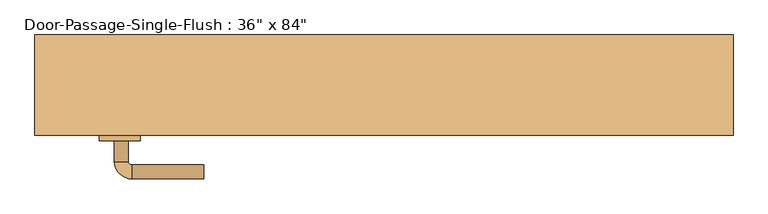
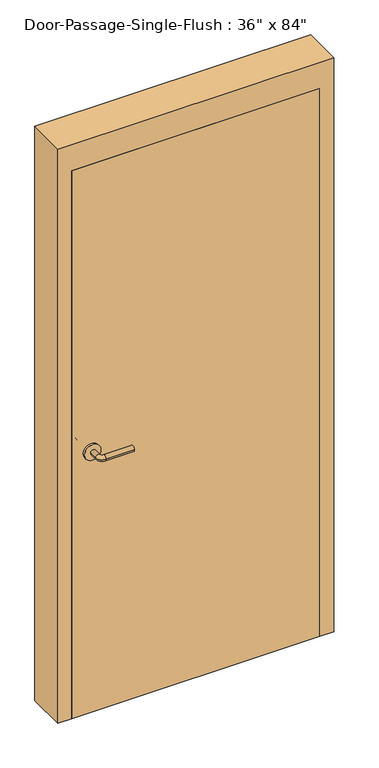
"""IFC4 building model written with IfcOpenShell, lengths in millimetres: door geometry."""

import ifcopenshell
import ifcopenshell.guid

model = None  # the IFC model being written
_history = None  # IfcOwnerHistory: only IFC2X3 demands one
_inside = {}  # id of a spatial element -> (the spatial element, [elements in it])
_under = {}  # id of a project, library or spatial element -> (it, [spatial elements below it])
_declared = {}  # id of a project -> (the project, [libraries it declares])
_typed = {}  # id of a type object -> (the type object, [elements of that type])
_made_of = {}  # id of a material, layer set ... -> (it, [elements and type objects made of it])


def new_model(schema):
    """Start an empty IFC model of exactly this schema.

    Asked for "IFC4X3", IfcOpenShell would pick the latest addendum, in which some entities
    have other attributes; the version numbers below select the first issue.
    IFC2X3 requires an IfcOwnerHistory on every rooted entity: one is made here for all.
    """
    global model, _history
    if schema == "IFC4X3":
        model = ifcopenshell.file(schema_version=(4, 3, 0, 0))
    else:
        model = ifcopenshell.file(schema=schema)
    _inside.clear()
    _under.clear()
    _declared.clear()
    _typed.clear()
    _made_of.clear()
    _history = None
    if model.schema == "IFC2X3":
        org = make("IfcOrganization", Name="unknown")
        user = make(
            "IfcPersonAndOrganization",
            ThePerson=make("IfcPerson", FamilyName="unknown"),
            TheOrganization=org,
        )
        app = make(
            "IfcApplication",
            ApplicationDeveloper=org,
            Version="unknown",
            ApplicationFullName="unknown",
            ApplicationIdentifier="unknown",
        )
        _history = make(
            "IfcOwnerHistory",
            OwningUser=user,
            OwningApplication=app,
            ChangeAction="ADDED",
            CreationDate=0,
        )
    return model


def make(cls, **values):
    """One entity of the class cls with the attributes given. An attribute that is None is left unset."""
    return model.create_entity(
        cls, **{name: value for name, value in values.items() if value is not None}
    )


def rooted(cls, **values):
    """An entity with a GlobalId (a new one), such as an element, a storey or a relation."""
    return make(cls, GlobalId=ifcopenshell.guid.new(), OwnerHistory=_history, **values)


def si_unit(unit_type, name, prefix=None):
    """IfcSIUnit, for example si_unit("LENGTHUNIT", "METRE", prefix="MILLI")."""
    return make("IfcSIUnit", UnitType=unit_type, Prefix=prefix, Name=name)


def assignment(units):
    """IfcUnitAssignment: the units of a project."""
    return None if units is None else make("IfcUnitAssignment", Units=units)


def point(xyz):
    """IfcCartesianPoint."""
    return None if xyz is None else make("IfcCartesianPoint", Coordinates=xyz)


def direction(xyz):
    """IfcDirection."""
    return None if xyz is None else make("IfcDirection", DirectionRatios=xyz)


def frame(location, z_axis=None, x_axis=None):
    """IfcAxis2Placement3D, a coordinate frame: its origin and axes. An axis left out is left unset."""
    return make(
        "IfcAxis2Placement3D",
        Location=point(location),
        Axis=direction(z_axis),
        RefDirection=direction(x_axis),
    )


def frame_2d(location, x_axis=None):
    """IfcAxis2Placement2D, a coordinate frame in the plane: its origin and x axis."""
    return make(
        "IfcAxis2Placement2D", Location=point(location), RefDirection=direction(x_axis)
    )


def origin():
    """The frame at (0, 0, 0) with its axes left unset."""
    return frame((0.0, 0.0, 0.0))


def origin_with_axes():
    """The frame at (0, 0, 0) with the z axis (0, 0, 1) and the x axis (1, 0, 0) written out."""
    return frame((0.0, 0.0, 0.0), z_axis=(0.0, 0.0, 1.0), x_axis=(1.0, 0.0, 0.0))


def place(relative_to, where):
    """IfcLocalPlacement: puts the frame where relative to a parent placement (None: the world)."""
    return make(
        "IfcLocalPlacement", PlacementRelTo=relative_to, RelativePlacement=where
    )


def context(
    kind, dimensions, precision=None, world=None, true_north=None, identifier=None
):
    """IfcGeometricRepresentationContext, for example the 3D "Model" context."""
    return make(
        "IfcGeometricRepresentationContext",
        ContextIdentifier=identifier,
        ContextType=kind,
        CoordinateSpaceDimension=dimensions,
        Precision=precision,
        WorldCoordinateSystem=world,
        TrueNorth=true_north,
    )


def project(units=None, contexts=None):
    """IfcProject with its units and contexts."""
    return rooted(
        "IfcProject",
        Name="project",
        RepresentationContexts=contexts,
        UnitsInContext=assignment(units),
    )


def spatial(cls, under=None, at=None, **own):
    """A site, building, storey or space (cls), placed at a placement, below another one or the project."""
    s = rooted(cls, ObjectPlacement=at, **own)
    if under is not None:
        _under.setdefault(under.id(), (under, []))[1].append(s)
    return s


def polyline(points):
    """IfcPolyline through the points."""
    return make("IfcPolyline", Points=[point(p) for p in points])


def circle_curve(where, radius):
    """IfcCircle in the frame where."""
    return make("IfcCircle", Position=where, Radius=radius)


def ellipse_curve(where, semi_axis1, semi_axis2):
    """IfcEllipse in the frame where."""
    return make(
        "IfcEllipse", Position=where, SemiAxis1=semi_axis1, SemiAxis2=semi_axis2
    )


def trimmed(basis, trim1, trim2, sense, master):
    """IfcTrimmedCurve: the piece of a basis curve between two trims."""
    return make(
        "IfcTrimmedCurve",
        BasisCurve=basis,
        Trim1=trim1,
        Trim2=trim2,
        SenseAgreement=sense,
        MasterRepresentation=master,
    )


def segment(curve, same_sense, transition):
    """IfcCompositeCurveSegment."""
    return make(
        "IfcCompositeCurveSegment",
        Transition=transition,
        SameSense=same_sense,
        ParentCurve=curve,
    )


def composite_curve(segments, self_intersect=None):
    """IfcCompositeCurve: segments joined end to end."""
    return make("IfcCompositeCurve", Segments=segments, SelfIntersect=self_intersect)


def outline(outer, holes=None, kind="AREA"):
    """IfcArbitraryClosedProfileDef: a profile drawn as a closed curve; with holes, ...WithVoids."""
    if holes is None:
        return make("IfcArbitraryClosedProfileDef", ProfileType=kind, OuterCurve=outer)
    return make(
        "IfcArbitraryProfileDefWithVoids",
        ProfileType=kind,
        OuterCurve=outer,
        InnerCurves=holes,
    )


def extrude(swept, where, along, depth):
    """IfcExtrudedAreaSolid: the profile swept, set in the frame where, extruded along a direction by depth."""
    return make(
        "IfcExtrudedAreaSolid",
        SweptArea=swept,
        Position=where,
        ExtrudedDirection=direction(along),
        Depth=depth,
    )


def faces_of(points, faces, orient=None, outer=None):
    """IfcFace entities. A face is a list of loops; a loop is a list of indices into points, from 0.

    orient and outer hold one flag for each loop. By default every Orientation is true, the
    first loop of a face is its IfcFaceOuterBound and the others are IfcFaceBound.
    """
    made = []
    for i, loops in enumerate(faces):
        bounds = []
        for j, loop in enumerate(loops):
            is_outer = j == 0 if outer is None else outer[i][j]
            bounds.append(
                make(
                    "IfcFaceOuterBound" if is_outer else "IfcFaceBound",
                    Bound=make("IfcPolyLoop", Polygon=[points[k] for k in loop]),
                    Orientation=True if orient is None else orient[i][j],
                )
            )
        made.append(make("IfcFace", Bounds=bounds))
    return made


def faceted_brep(points, faces, orient=None, outer=None, voids=None):
    """IfcFacetedBrep: a solid bounded by flat faces; with voids (closed shells), ...WithVoids."""
    shared = [point(p) for p in points]
    hull = make("IfcClosedShell", CfsFaces=faces_of(shared, faces, orient, outer))
    if voids is None:
        return make("IfcFacetedBrep", Outer=hull)
    return make(
        "IfcFacetedBrepWithVoids",
        Outer=hull,
        Voids=[
            make(cls, CfsFaces=faces_of(shared, fs, o, b)) for cls, fs, o, b in voids
        ],
    )


def shape(context_of_items, identifier, shape_type, items):
    """IfcShapeRepresentation: the items that make up one representation, for example the "Body"."""
    return make(
        "IfcShapeRepresentation",
        ContextOfItems=context_of_items,
        RepresentationIdentifier=identifier,
        RepresentationType=shape_type,
        Items=items,
    )


def source(mapping_origin, context_of_items, identifier, shape_type, items):
    """IfcRepresentationMap: a shape defined once, which mapped items show again and again."""
    return make(
        "IfcRepresentationMap",
        MappingOrigin=mapping_origin,
        MappedRepresentation=shape(context_of_items, identifier, shape_type, items),
    )


def transform(
    local_origin,
    x_axis=None,
    y_axis=None,
    z_axis=None,
    scale=None,
    scale2=None,
    scale3=None,
    uniform=True,
):
    """IfcCartesianTransformationOperator3D, or its non-uniform kind. x_axis, y_axis, z_axis: its Axis1, 2, 3."""
    if uniform:
        return make(
            "IfcCartesianTransformationOperator3D",
            Axis1=direction(x_axis),
            Axis2=direction(y_axis),
            LocalOrigin=point(local_origin),
            Scale=scale,
            Axis3=direction(z_axis),
        )
    return make(
        "IfcCartesianTransformationOperator3DnonUniform",
        Axis1=direction(x_axis),
        Axis2=direction(y_axis),
        LocalOrigin=point(local_origin),
        Scale=scale,
        Axis3=direction(z_axis),
        Scale2=scale2,
        Scale3=scale3,
    )


def mapped(mapping_source, mapping_target):
    """IfcMappedItem: shows the shape of a source again, moved by a transform."""
    return make(
        "IfcMappedItem", MappingSource=mapping_source, MappingTarget=mapping_target
    )


def made_of(thing, what):
    """Note that an element or type object is made of a material, layer set ...; save() writes the relation."""
    if what is not None:
        _made_of.setdefault(what.id(), (what, []))[1].append(thing)
    return thing


def element(
    cls,
    number,
    at=None,
    inside=None,
    cuts=None,
    type_object=None,
    material=None,
    context=None,
    identifier="Body",
    shape_type=None,
    held_by="IfcProductDefinitionShape",
    body=None,
    shapes=None,
    **own,
):
    """One element of the class cls, such as IfcWall. Its Tag is "e" and its number.

    at: its placement. inside: the storey or other place that contains it. cuts: it is an
    opening in that element (IfcRelVoidsElement). A single representation is given by context,
    identifier, shape_type and body (its items); several are given by shapes. held_by: the class
    of the entity that holds the representations. save() writes the other relations.
    """
    e = rooted(cls, Tag="e%d" % number, ObjectPlacement=at, **own)
    if body is not None:
        shapes = [shape(context, identifier, shape_type, body)]
    if shapes is not None:
        e.Representation = make(held_by, Representations=shapes)
    if inside is not None:
        _inside.setdefault(inside.id(), (inside, []))[1].append(e)
    if cuts is not None:
        rooted(
            "IfcRelVoidsElement", RelatingBuildingElement=cuts, RelatedOpeningElement=e
        )
    if type_object is not None:
        _typed.setdefault(type_object.id(), (type_object, []))[1].append(e)
    return made_of(e, material)


def aggregate(whole, parts):
    """IfcRelAggregates: a whole, such as a stair, and the parts it consists of."""
    return rooted("IfcRelAggregates", RelatingObject=whole, RelatedObjects=parts)


def save(model, path):
    """Write the relations noted so far, then the file.

    IfcRelAggregates (storeys below a building ...), IfcRelContainedInSpatialStructure (elements
    in a storey), IfcRelDefinesByType, IfcRelAssociatesMaterial and IfcRelDeclares: one each for
    every whole, place, type object, material and project.
    """
    for whole, parts in _under.values():
        aggregate(whole, parts)
    for where, things in _inside.values():
        rooted(
            "IfcRelContainedInSpatialStructure",
            RelatedElements=things,
            RelatingStructure=where,
        )
    for kind, things in _typed.values():
        rooted("IfcRelDefinesByType", RelatedObjects=things, RelatingType=kind)
    for what, things in _made_of.values():
        rooted("IfcRelAssociatesMaterial", RelatedObjects=things, RelatingMaterial=what)
    for by, libraries in _declared.values():
        rooted("IfcRelDeclares", RelatingContext=by, RelatedDefinitions=libraries)
    model.write(path)


def plane_surface(at):
    """IfcPlane: the flat surface through the origin of the frame at, square to its z axis."""
    return make("IfcPlane", Position=at)


def cylinder_surface(at, radius):
    """IfcCylindricalSurface: all points at the distance radius from the z axis of the frame at."""
    return make("IfcCylindricalSurface", Position=at, Radius=radius)


def revolved_surface(curve, axis_point, axis_direction):
    """IfcSurfaceOfRevolution: the curve turned about the line through axis_point along axis_direction."""
    return make(
        "IfcSurfaceOfRevolution",
        SweptCurve=make("IfcArbitraryOpenProfileDef", ProfileType="CURVE", Curve=curve),
        AxisPosition=make("IfcAxis1Placement", Location=point(axis_point), Axis=direction(axis_direction)),
    )


def advanced_brep(points, edges, surfaces, faces):
    """IfcAdvancedBrep: a solid bounded by faces that lie on surfaces and meet in shared edges.

    An edge is (start, end): straight between two places in points (the first is 0);
    or (start, end, curve); or (start, end, curve, False) where it runs against its curve.
    A face is (place in surfaces, loops), or (place, loops, False) where it looks against
    its surface's normal. A loop lists edges by number (the first is 1), with a minus sign
    where the edge is run from its end to its start. The first loop is the outer one.
    """
    corners = [point(p) for p in points]
    vertices = [make("IfcVertexPoint", VertexGeometry=c) for c in corners]
    made = []
    for start, end, *more in edges:
        made.append(
            make(
                "IfcEdgeCurve",
                EdgeStart=vertices[start],
                EdgeEnd=vertices[end],
                EdgeGeometry=more[0] if more else make("IfcPolyline", Points=[corners[start], corners[end]]),
                SameSense=more[1] if len(more) > 1 else True,
            )
        )
    hull = []
    for where, loops, *sense in faces:
        bounds = []
        for j, loop in enumerate(loops):
            ring = [make("IfcOrientedEdge", EdgeElement=made[abs(k) - 1], Orientation=k > 0) for k in loop]
            bounds.append(
                make(
                    "IfcFaceOuterBound" if j == 0 else "IfcFaceBound",
                    Bound=make("IfcEdgeLoop", EdgeList=ring),
                    Orientation=True,
                )
            )
        hull.append(make("IfcAdvancedFace", Bounds=bounds, FaceSurface=surfaces[where], SameSense=sense[0] if sense else True))
    return make("IfcAdvancedBrep", Outer=make("IfcClosedShell", CfsFaces=hull))


def door_5b314290(model_context):
    return source(origin(), model_context, "Body", "SolidModel", [
        advanced_brep(
        [(-392.190625, 1.65, 1016.0), (-372.190625, 1.65, 1016.0), (-392.190625, 31.65, 1016.0), (-372.190625, 31.65, 1016.0), (-367.190625, 36.65, 1016.0), (-367.190625, 56.65, 1016.0), (-262.190625, 56.65, 1016.0), (-262.190625, 36.65, 1016.0)],
        [
            (0, 1, circle_curve(frame((-382.190625, 1.65, 1016.0), z_axis=(0.0, -1.0, 0.0), x_axis=(1.0, 0.0, 0.0)), 10.0)),
            (1, 0, circle_curve(frame((-382.190625, 1.65, 1016.0), z_axis=(0.0, -1.0, 0.0), x_axis=(1.0, 0.0, 0.0)), 10.0)),
            (0, 2),
            (2, 3, circle_curve(frame((-382.190625, 31.65, 1016.0), z_axis=(0.0, -1.0, 0.0), x_axis=(1.0, 0.0, 0.0)), 10.0)),
            (3, 1),
            (3, 2, circle_curve(frame((-382.190625, 31.65, 1016.0), z_axis=(0.0, -1.0, 0.0), x_axis=(1.0, 0.0, 0.0)), 10.0)),
            (4, 3, circle_curve(frame((-367.190625, 31.65, 1016.0), z_axis=(0.0, 0.0, 1.0), x_axis=(-1.0, 0.0, 0.0)), 5.0)),
            (2, 5, circle_curve(frame((-367.190625, 31.65, 1016.0), z_axis=(0.0, 0.0, -1.0), x_axis=(-1.0, 0.0, 0.0)), 25.0)),
            (5, 4, circle_curve(frame((-367.190625, 46.65, 1016.0), z_axis=(-1.0, 0.0, 0.0), x_axis=(0.0, -1.0, 0.0)), 10.0)),
            (4, 5, circle_curve(frame((-367.190625, 46.65, 1016.0), z_axis=(-1.0, 0.0, 0.0), x_axis=(0.0, -1.0, 0.0)), 10.0)),
            (6, 7, circle_curve(frame((-262.190625, 46.65, 1016.0), z_axis=(1.0, 0.0, 0.0), x_axis=(0.0, -1.0, 0.0)), 10.0)),
            (7, 6, circle_curve(frame((-262.190625, 46.65, 1016.0), z_axis=(1.0, 0.0, 0.0), x_axis=(0.0, -1.0, 0.0)), 10.0)),
            (5, 6),
            (7, 4),
        ],
        [
            plane_surface(frame((-382.190625, 1.65, 1016.0), z_axis=(0.0, -1.0, 0.0), x_axis=(0.0, 0.0, 1.0))),
            cylinder_surface(frame((-382.190625, 1.65, 1016.0), z_axis=(0.0, -1.0, 0.0), x_axis=(1.0, 0.0, 0.0)), 10.0),
            revolved_surface(trimmed(ellipse_curve(frame((-382.190625, 31.65, 1016.0), z_axis=(0.0, -1.0, 0.0), x_axis=(1.0, 0.0, 0.0)), 10.0, 10.0), [point((-392.190625, 31.65, 1016.0))], [point((-372.190625, 31.65, 1016.0))], True, "CARTESIAN"), (-367.190625, 31.65, 1016.0), (0.0, 0.0, -1.0)),
            revolved_surface(trimmed(ellipse_curve(frame((-382.190625, 31.65, 1016.0), z_axis=(0.0, -1.0, 0.0), x_axis=(1.0, 0.0, 0.0)), 10.0, 10.0), [point((-372.190625, 31.65, 1016.0))], [point((-392.190625, 31.65, 1016.0))], True, "CARTESIAN"), (-367.190625, 31.65, 1016.0), (0.0, 0.0, -1.0)),
            plane_surface(frame((-262.190625, 46.65, 1016.0), z_axis=(1.0, 0.0, 0.0), x_axis=(0.0, 0.0, 1.0))),
            cylinder_surface(frame((-367.190625, 46.65, 1016.0), z_axis=(-1.0, 0.0, 0.0), x_axis=(0.0, -1.0, 0.0)), 10.0),
        ],
        [
            (0, [[1, 2]]),
            (1, [[-1, 3, 4, 5]]),
            (1, [[-2, -5, 6, -3]]),
            (2, [[7, -4, 8, 9]]),
            (3, [[-8, -6, -7, 10]]),
            (4, [[11, 12]]),
            (5, [[-9, 13, -12, 14]]),
            (5, [[-10, -14, -11, -13]]),
        ],
    ),
        extrude(outline(composite_curve([segment(trimmed(circle_curve(frame_2d((1016.0, -384.690625)), 30.0), [point((1016.0, -414.690625))], [point((1016.0, -354.690625))], False, "CARTESIAN"), True, "CONTINUOUS"), segment(trimmed(circle_curve(frame_2d((1016.0, -384.690625)), 30.0), [point((1016.0, -354.690625))], [point((1016.0, -414.690625))], False, "CARTESIAN"), True, "CONTINUOUS")], self_intersect=False)), frame((0.0, -6.35, 0.0), z_axis=(0.0, 1.0, 0.0), x_axis=(0.0, 0.0, 1.0)), (0.0, 0.0, 1.0), 8.0),
        advanced_brep(
        [(-392.190625, -58.8, 1016.0), (-372.190625, -58.8, 1016.0), (-372.190625, -88.8, 1016.0), (-392.190625, -88.8, 1016.0), (-367.190625, -93.8, 1016.0), (-367.190625, -113.8, 1016.0), (-262.190625, -113.8, 1016.0), (-262.190625, -93.8, 1016.0)],
        [
            (0, 1, circle_curve(frame((-382.190625, -58.8, 1016.0), z_axis=(0.0, 1.0, 0.0), x_axis=(1.0, 0.0, 0.0)), 10.0)),
            (1, 0, circle_curve(frame((-382.190625, -58.8, 1016.0), z_axis=(0.0, 1.0, 0.0), x_axis=(1.0, 0.0, 0.0)), 10.0)),
            (1, 2),
            (2, 3, circle_curve(frame((-382.190625, -88.8, 1016.0), z_axis=(0.0, 1.0, 0.0), x_axis=(1.0, 0.0, 0.0)), 10.0)),
            (3, 0),
            (3, 2, circle_curve(frame((-382.190625, -88.8, 1016.0), z_axis=(0.0, 1.0, 0.0), x_axis=(1.0, 0.0, 0.0)), 10.0)),
            (4, 5, circle_curve(frame((-367.190625, -103.8, 1016.0), z_axis=(-1.0, 0.0, 0.0), x_axis=(0.0, 1.0, 0.0)), 10.0)),
            (5, 3, circle_curve(frame((-367.190625, -88.8, 1016.0), z_axis=(0.0, 0.0, -1.0), x_axis=(-1.0, 0.0, 0.0)), 25.0)),
            (2, 4, circle_curve(frame((-367.190625, -88.8, 1016.0), z_axis=(0.0, 0.0, 1.0), x_axis=(-1.0, 0.0, 0.0)), 5.0)),
            (5, 4, circle_curve(frame((-367.190625, -103.8, 1016.0), z_axis=(-1.0, 0.0, 0.0), x_axis=(0.0, 1.0, 0.0)), 10.0)),
            (6, 7, circle_curve(frame((-262.190625, -103.8, 1016.0), z_axis=(1.0, 0.0, 0.0), x_axis=(0.0, 1.0, 0.0)), 10.0)),
            (7, 6, circle_curve(frame((-262.190625, -103.8, 1016.0), z_axis=(1.0, 0.0, 0.0), x_axis=(0.0, 1.0, 0.0)), 10.0)),
            (4, 7),
            (6, 5),
        ],
        [
            plane_surface(frame((-382.190625, -58.8, 1016.0), z_axis=(0.0, 1.0, 0.0), x_axis=(0.0, 0.0, 1.0))),
            cylinder_surface(frame((-382.190625, -58.8, 1016.0), z_axis=(0.0, 1.0, 0.0), x_axis=(1.0, 0.0, 0.0)), 10.0),
            revolved_surface(trimmed(ellipse_curve(frame((-382.190625, -88.8, 1016.0), z_axis=(0.0, -1.0, 0.0), x_axis=(1.0, 0.0, 0.0)), 10.0, 10.0), [point((-392.190625, -88.8, 1016.0))], [point((-372.190625, -88.8, 1016.0))], True, "CARTESIAN"), (-367.190625, -88.8, 1016.0), (0.0, 0.0, -1.0)),
            revolved_surface(trimmed(ellipse_curve(frame((-382.190625, -88.8, 1016.0), z_axis=(0.0, -1.0, 0.0), x_axis=(1.0, 0.0, 0.0)), 10.0, 10.0), [point((-372.190625, -88.8, 1016.0))], [point((-392.190625, -88.8, 1016.0))], True, "CARTESIAN"), (-367.190625, -88.8, 1016.0), (0.0, 0.0, -1.0)),
            plane_surface(frame((-262.190625, -103.8, 1016.0), z_axis=(1.0, 0.0, 0.0), x_axis=(0.0, 0.0, 1.0))),
            cylinder_surface(frame((-367.190625, -103.8, 1016.0), z_axis=(-1.0, 0.0, 0.0), x_axis=(0.0, 1.0, 0.0)), 10.0),
        ],
        [
            (0, [[1, 2]]),
            (1, [[3, 4, 5, -2]]),
            (1, [[-5, 6, -3, -1]]),
            (2, [[7, 8, -4, 9]]),
            (3, [[10, -9, -6, -8]]),
            (4, [[11, 12]]),
            (5, [[13, -11, 14, -7]]),
            (5, [[-14, -12, -13, -10]]),
        ],
    ),
        extrude(outline(composite_curve([segment(trimmed(circle_curve(frame_2d((1016.0, -384.690625)), 30.0), [point((1016.0, -414.690625))], [point((1016.0, -354.690625))], False, "CARTESIAN"), True, "CONTINUOUS"), segment(trimmed(circle_curve(frame_2d((1016.0, -384.690625)), 30.0), [point((1016.0, -354.690625))], [point((1016.0, -414.690625))], False, "CARTESIAN"), True, "CONTINUOUS")], self_intersect=False)), frame((0.0, -58.8, 0.0), z_axis=(0.0, 1.0, 0.0), x_axis=(0.0, 0.0, 1.0)), (0.0, 0.0, 1.0), 8.0),
        faceted_brep([(457.2, -1.5875, 0.0), (441.325, -1.5875, 0.0), (441.325, 46.0375, 0.0), (457.2, 46.0375, 0.0), (457.2, 95.25, 0.0), (508.0, 95.25, 0.0), (508.0, -50.8, 0.0), (457.2, -50.8, 0.0), (457.2, -50.8, 2133.6), (457.2, -1.5875, 2133.6), (508.0, -50.8, 2235.2), (-508.0, -50.8, 2235.2), (-508.0, -50.8, 0.0), (-457.2, -50.8, 0.0), (-457.2, -50.8, 2133.6), (508.0, 95.25, 2235.2), (457.2, 95.25, 2133.6), (-457.2, 95.25, 2133.6), (-457.2, 95.25, 0.0), (-508.0, 95.25, 0.0), (-508.0, 95.25, 2235.2), (457.2, 46.0375, 2133.6), (441.325, 46.0375, 2117.725), (-441.325, 46.0375, 2117.725), (-441.325, 46.0375, 0.0), (-457.2, 46.0375, 0.0), (-457.2, 46.0375, 2133.6), (441.325, -1.5875, 2117.725), (-457.2, -1.5875, 2133.6), (-457.2, -1.5875, 0.0), (-441.325, -1.5875, 0.0), (-441.325, -1.5875, 2117.725)], [[[0, 1, 2, 3, 4, 5, 6, 7]], [[7, 8, 9, 0]], [[6, 10, 11, 12, 13, 14, 8, 7]], [[5, 15, 10, 6]], [[4, 16, 17, 18, 19, 20, 15, 5]], [[3, 21, 16, 4]], [[2, 22, 23, 24, 25, 26, 21, 3]], [[1, 27, 22, 2]], [[0, 9, 28, 29, 30, 31, 27, 1]], [[8, 14, 28, 9]], [[16, 21, 26, 17]], [[22, 27, 31, 23]], [[12, 19, 18, 25, 24, 30, 29, 13]], [[13, 29, 28, 14]], [[11, 20, 19, 12]], [[17, 26, 25, 18]], [[23, 31, 30, 24]], [[15, 20, 11, 10]]]),
        extrude(outline(polyline([(457.2, -6.35), (457.2, -50.8), (-457.2, -50.8), (-457.2, -6.35), (457.2, -6.35)])), origin_with_axes(), (0.0, 0.0, 1.0), 2133.6),
    ])


if __name__ == "__main__":
    model = new_model("IFC4")
    model_context = context("Model", 3, world=origin())
    ifc_project = project(units=[si_unit("LENGTHUNIT", "METRE", prefix="MILLI")], contexts=[model_context])
    site = spatial("IfcSite", under=ifc_project)
    building = spatial("IfcBuilding", under=site)
    placement = place(None, origin())
    door_shape = door_5b314290(model_context)
    element("IfcDoor", 1, ObjectType="Door-Passage-Single-Flush : 36\" x 84\"", at=placement, inside=building, context=model_context, shape_type="MappedRepresentation", body=[
        mapped(door_shape, transform((0.0, 0.0, 0.0), x_axis=(1.0, 0.0, 0.0), y_axis=(0.0, 1.0, 0.0), z_axis=(0.0, 0.0, 1.0))),
    ])
    save(model, "model.ifc")

# Revit data of these elements
# Type "Door-Passage-Single-Flush : 36\" x 84\""
#   Type Mark = "35"
#   Assembly Code = "B2030200"
#   Analytic Construction = "Wooden"
#   Thickness = 0' - 1 3/4"
#   Thermal Resistance (R) = 2.5876 (h·ft²·°F)/BTU
#   Swing Angle [instance default] = 90.00°
#   Strike Height = 3' - 4"
#   Rough Width [instance default] = 3' - 4"
#   Rough Height [instance default] = 7' - 4"
#   MF Opening Height [instance default] = 0' - 4"
#   MF Opening Width [instance default] = 0' - 4"
#   Inset Calculate [instance default] = 0' - 4"
#   Masonry Inset [instance default] = 0' - 1"
#   Height = 7' - 0"
#   Width = 3' - 0"
#   Heat Transfer Coefficient (U) = 0.3865 BTU/(h·ft²·°F)
#   Masonry Frame Depth = 0' - 5 3/4"
#   Masonry Frame [instance default] = yes
#   Function = 1
#   Dry Wall Frame [instance default] = no
#   Panel Material = Wood - Birch
#   Frame Material = Metal - Paint Finish - Grey
#   Door Handle Material = Aluminum
#   Visual Light Transmittance = 0
#   Solar Heat Gain Coefficient = 0
#   Wall Closure = (empty or 0)
# Element 1 (IfcDoor, "Door-Passage-Single-Flush : 36\" x 84\"")
#   Materials on its faces: "Aluminum", "Metal - Paint Finish - Grey", "Wood - Birch"
# Materials
#   "Wood - Birch": class "Wood", colour RGB 166 116 52, transparency 0, Cost = 0
#   "Metal - Paint Finish - Grey": class "Paint", colour RGB 104 104 104, transparency 0, Cost = 0
#   "Aluminum": class "Metal", colour RGB 247 247 247, transparency 0, Description = "Aluminum 6061", Cost = 0
